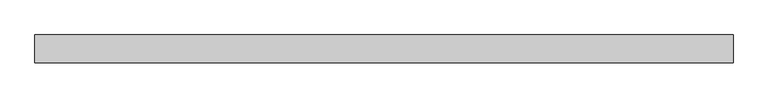
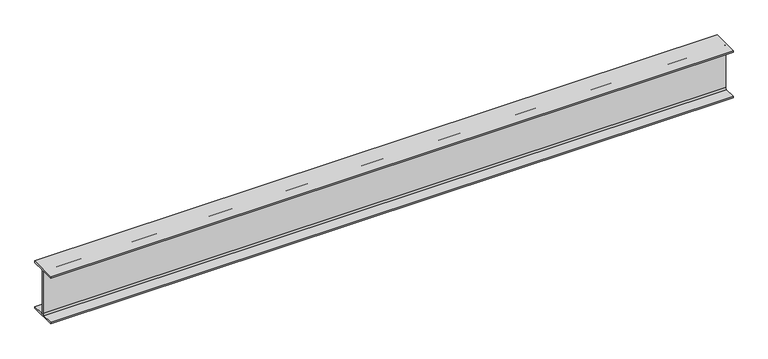
"""IFC4 building model written with IfcOpenShell, lengths in millimetres: beam geometry, Steel Beam_H-KSD3502 : H_SB_ASB_H-250x125x6x9."""

from ifc_helpers import new_model, si_unit, point, frame, frame_2d, origin, place, context, project, spatial, polyline, circle_curve, trimmed, segment, composite_curve, outline, extrude, source, transform, mapped, element, save


def beam_10e9c193(model_context):
    return source(origin(), model_context, "Body", "SweptSolid", [
        extrude(outline(composite_curve([segment(polyline([(82.5, -141.5), (82.5, -151.7), (-82.5, -151.7), (-82.5, -141.5), (-11.9, -141.5)]), True, "CONTINUOUS"), segment(trimmed(circle_curve(frame_2d((-11.9, -132.6)), 8.9), [point((-11.9, -141.5))], [point((-3.0, -132.6))], True, "CARTESIAN"), True, "CONTINUOUS"), segment(polyline([(-3.0, -132.6), (-3.0, 132.6)]), True, "CONTINUOUS"), segment(trimmed(circle_curve(frame_2d((-11.9, 132.6)), 8.9), [point((-3.0, 132.6))], [point((-11.9, 141.5))], True, "CARTESIAN"), True, "CONTINUOUS"), segment(polyline([(-11.9, 141.5), (-82.5, 141.5), (-82.5, 151.7), (82.5, 151.7), (82.5, 141.5), (11.9, 141.5)]), True, "CONTINUOUS"), segment(trimmed(circle_curve(frame_2d((11.9, 132.6)), 8.9), [point((11.9, 141.5))], [point((3.0, 132.6))], True, "CARTESIAN"), True, "CONTINUOUS"), segment(polyline([(3.0, 132.6), (3.0, -132.6)]), True, "CONTINUOUS"), segment(trimmed(circle_curve(frame_2d((11.9, -132.6)), 8.9), [point((3.0, -132.6))], [point((11.9, -141.5))], True, "CARTESIAN"), True, "CONTINUOUS"), segment(polyline([(11.9, -141.5), (82.5, -141.5)]), True, "CONTINUOUS")], self_intersect=False)), frame((-2029.8, 0.0, 0.0), z_axis=(1.0, 0.0, 0.0), x_axis=(0.0, 1.0, 0.0)), (0.0, 0.0, 1.0), 4142.0999994),
    ])


if __name__ == "__main__":
    model = new_model("IFC4")
    model_context = context("Model", 3, world=origin())
    ifc_project = project(units=[si_unit("LENGTHUNIT", "METRE", prefix="MILLI")], contexts=[model_context])
    site = spatial("IfcSite", under=ifc_project)
    building = spatial("IfcBuilding", under=site)
    placement = place(None, origin())
    beam_shape = beam_10e9c193(model_context)
    element("IfcBeam", 1, ObjectType="Steel Beam_H-KSD3502 : H_SB_ASB_H-250x125x6x9", at=placement, inside=building, context=model_context, shape_type="MappedRepresentation", body=[
        mapped(beam_shape, transform((0.0, 0.0, 0.0), x_axis=(1.0, 0.0, 0.0), y_axis=(0.0, 1.0, 0.0), z_axis=(0.0, 0.0, 1.0))),
    ])
    save(model, "model.ifc")

# Revit data of these elements
# Type "Steel Beam_H-KSD3502 : H_SB_ASB_H-250x125x6x9"
#   Width = 12.5 cm
#   Web Thickness = 0.6 cm
#   Web Fillet = 1.2 cm
#   Warping Constant = 42539.8 cm⁶
#   Torsional Moment of Inertia = 7.8102 cm⁴
#   Torsional Modulus = 1.0 cm³
#   Section Area = 37.66 cm²
#   Plastic Modulus weak axis = 73.1 cm³
#   Plastic Modulus strong axis = 366.0 cm³
#   Perimeter = 0.97 m²/m
#   Nominal Weight = 29.60 kgf/m
#   Moment of Inertia weak axis = 294.00 cm⁴
#   Moment of Inertia strong axis = 4050.00 cm⁴
#   Height = 25.0 cm
#   Flange Thickness = 0.9 cm
#   Elastic Modulus weak axis = 47.0 cm³
#   Elastic Modulus strong axis = 324.0 cm³
#   Centroid Vertical = 12.5 cm
#   Centroid Horizontal = 6.25 cm
#   Length [instance default] = 1.5240 m
#   Structural Material [instance default] = Steel, 45-345
#   Assembly Code = ""
# Element 1 (IfcBeam, "Steel Beam_H-KSD3502 : H_SB_ASB_H-250x125x6x9")
#   Structural Material = none
# Materials
#   "Steel, 45-345": class "Metal", colour RGB 189 187 185, transparency 0, Description = "Steel 345 MPa", Cost = 0
